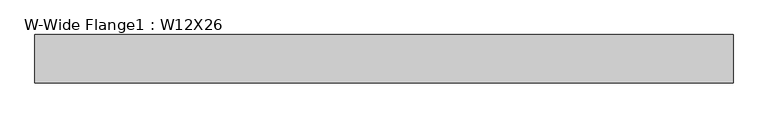
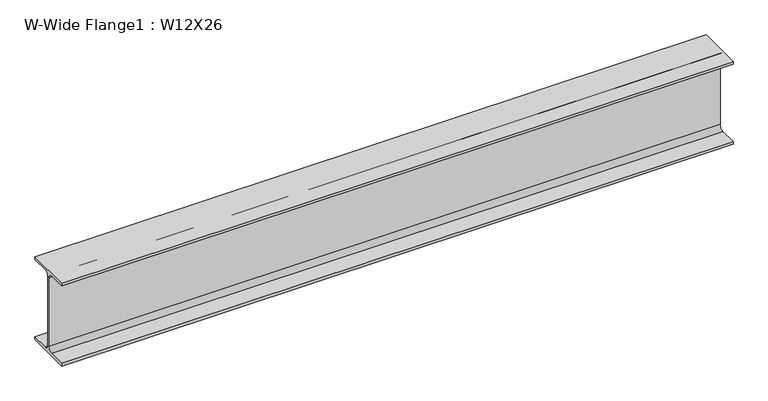
"""IFC4 building model written with IfcOpenShell, lengths in millimetres: beam geometry, W-Wide Flange1 : W12X26."""

from ifc_helpers import new_model, si_unit, point, frame, frame_2d, origin, place, context, project, spatial, polyline, circle_curve, trimmed, segment, composite_curve, outline, extrude, source, transform, mapped, element, save


def w_wide_flange1_w12x26_1eedce2b(model_context):
    return source(origin(), model_context, "Body", "SweptSolid", [
        extrude(outline(composite_curve([segment(polyline([(82.423, -145.288), (82.423, -154.94), (-82.423, -154.94), (-82.423, -145.288), (-20.2565, -145.288)]), True, "CONTINUOUS"), segment(trimmed(circle_curve(frame_2d((-20.2565, -127.9525)), 17.3355), [point((-20.2565, -145.288))], [point((-2.921, -127.9525))], True, "CARTESIAN"), True, "CONTINUOUS"), segment(polyline([(-2.921, -127.9525), (-2.921, 127.9525)]), True, "CONTINUOUS"), segment(trimmed(circle_curve(frame_2d((-20.2565, 127.9525)), 17.3355), [point((-2.921, 127.9525))], [point((-20.2565, 145.288))], True, "CARTESIAN"), True, "CONTINUOUS"), segment(polyline([(-20.2565, 145.288), (-82.423, 145.288), (-82.423, 154.94), (82.423, 154.94), (82.423, 145.288), (20.2565, 145.288)]), True, "CONTINUOUS"), segment(trimmed(circle_curve(frame_2d((20.2565, 127.9525)), 17.3355), [point((20.2565, 145.288))], [point((2.921, 127.9525))], True, "CARTESIAN"), True, "CONTINUOUS"), segment(polyline([(2.921, 127.9525), (2.921, -127.9525)]), True, "CONTINUOUS"), segment(trimmed(circle_curve(frame_2d((20.2565, -127.9525)), 17.3355), [point((2.921, -127.9525))], [point((20.2565, -145.288))], True, "CARTESIAN"), True, "CONTINUOUS"), segment(polyline([(20.2565, -145.288), (82.423, -145.288)]), True, "CONTINUOUS")], self_intersect=False)), frame((-1180.3322818, 0.0, 0.0), z_axis=(1.0, 0.0, 0.0), x_axis=(0.0, 1.0, 0.0)), (0.0, 0.0, 1.0), 2380.1242233),
    ])


if __name__ == "__main__":
    model = new_model("IFC4")
    model_context = context("Model", 3, world=origin())
    ifc_project = project(units=[si_unit("LENGTHUNIT", "METRE", prefix="MILLI")], contexts=[model_context])
    site = spatial("IfcSite", under=ifc_project)
    building = spatial("IfcBuilding", under=site)
    placement = place(None, origin())
    w_wide_flange1_w12x26_shape = w_wide_flange1_w12x26_1eedce2b(model_context)
    element("IfcBeam", 1, ObjectType="W-Wide Flange1 : W12X26", at=placement, inside=building, context=model_context, shape_type="MappedRepresentation", body=[
        mapped(w_wide_flange1_w12x26_shape, transform((0.0, 0.0, 0.0), x_axis=(1.0, 0.0, 0.0), y_axis=(0.0, 1.0, 0.0), z_axis=(0.0, 0.0, 1.0))),
    ])
    save(model, "model.ifc")

# Revit data of these elements
# Type "W-Wide Flange1 : W12X26"
#   Assembly Code = "B10"
#   W = 26
#   Start Extension Calculation [instance default] = 10' - 0"
#   Start Extension [instance default] = -0' - 0 1/2"
#   End Extension Calculation [instance default] = 10' - 0"
#   End Extension [instance default] = -0' - 0 1/2"
#   Length [instance default] = 5' - 0"
#   bf = 0' - 6.49"
#   d = 1' - 0.2"
#   k = 0' - 1 1/16"
#   k2 = 0' - 0.6825"
#   tf = 0' - 0.38"
#   tw = 0' - 0.23"
#   A = 0.053125 SF
#   Structural Material [instance default] = Metal - Steel - ASTM A992
# Element 1 (IfcBeam, "W-Wide Flange1 : W12X26")
#   Materials on its faces: "Metal - Steel - ASTM A992"
# Materials
#   "Metal - Steel - ASTM A992": class "Metal", colour RGB 199 199 199, transparency 0
